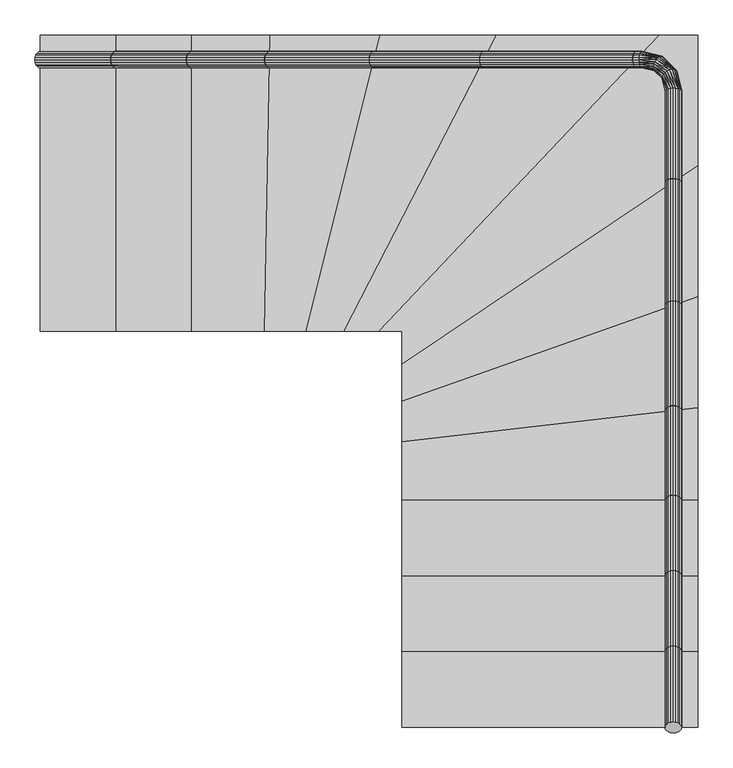
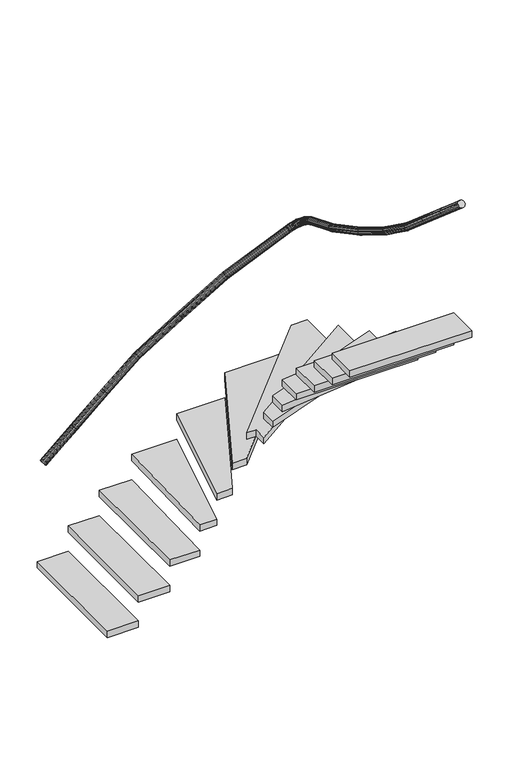
"""IFC4 building model written with IfcOpenShell, lengths in millimetres: stair geometry, 0_3d_modell."""

from ifc_helpers import new_model, si_unit, frame, origin, origin_with_axes, place, context, project, spatial, polyline, outline, extrude, faceted_brep, source, transform, mapped, element, save


def stair_1cae02e6(model_context):
    return source(origin(), model_context, "Body", "SolidModel", [
        extrude(outline(polyline([(1116.9018591, 1121.5036957), (2016.9018591, 1724.0707938), (2016.9018591, 1326.2140709), (1116.9018591, 1007.5896473), (1116.9018591, 1121.5036957)])), frame((0.0, 0.0, 1390.0), z_axis=(0.0, 0.0, 1.0), x_axis=(1.0, 0.0, 0.0)), (0.0, 0.0, 1.0), 50.0),
        extrude(outline(polyline([(1116.9018591, 476.9018591), (2016.9018591, 476.9018591), (2016.9018591, 246.9018591), (1116.9018591, 246.9018591), (1116.9018591, 476.9018591)])), frame((0.0, 0.0, 2184.2857143), z_axis=(0.0, 0.0, 1.0), x_axis=(1.0, 0.0, 0.0)), (0.0, 0.0, 1.0), 50.0),
        extrude(outline(polyline([(1.2235871, -7.9923214), (0.0, 0.0), (1.2235871, 7.9923214), (4.7745751, 15.2022986), (10.3053687, 20.9241691), (17.2745751, 24.5978359), (25.0, 25.8636953), (32.7254248, 24.5978359), (39.6946313, 20.9241691), (45.2254248, 15.2022986), (48.7764129, 7.9923214), (50.0, 0.0), (48.7764129, -7.9923214), (45.2254248, -15.2022986), (39.6946313, -20.924169), (32.7254248, -24.5978359), (25.0, -25.8636953), (17.2745751, -24.5978359), (10.3053687, -20.924169), (4.7745751, -15.2022986), (1.2235871, -7.9923214)])), frame((16.9018591, 2071.5036957, 869.5592366), z_axis=(0.7569287102857587, 0.0, 0.6534974579484897), x_axis=(0.0, -1.0, 0.0)), (0.0, 0.0, 1.0), 303.8595272),
        extrude(outline(polyline([(939.4821841, 1221.5036957), (1403.2627923, 2121.5036957), (1898.8029965, 2121.5036957), (1046.9018591, 1221.5036957), (939.4821841, 1221.5036957)])), frame((0.0, 0.0, 992.8571429), z_axis=(0.0, 0.0, 1.0), x_axis=(1.0, 0.0, 0.0)), (0.0, 0.0, 1.0), 50.0),
        faceted_brep([(1965.678272, 1303.6496314, 2465.062536), (1966.9018591, 1299.6620356, 2458.1306652), (1965.678272, 1295.6744399, 2451.1987943), (1962.127284, 1292.0771778, 2444.9454632), (1956.5964904, 1289.2223744, 2439.9827916), (1949.627284, 1287.3894778, 2436.7965603), (1941.9018591, 1286.7579047, 2435.6986598), (1934.1764343, 1287.3894778, 2436.7965603), (1927.2072278, 1289.2223744, 2439.9827916), (1921.6764343, 1292.0771778, 2444.9454632), (1918.1254462, 1295.6744399, 2451.1987943), (1916.9018591, 1299.6620356, 2458.1306652), (1918.1254462, 1303.6496314, 2465.062536), (1921.6764343, 1307.2468935, 2471.3158671), (1927.2072278, 1310.1016969, 2476.2785387), (1934.1764343, 1311.9345935, 2479.46477), (1941.9018591, 1312.5661666, 2480.5626705), (1949.627284, 1311.9345935, 2479.46477), (1956.5964904, 1310.1016969, 2476.2785387), (1962.127284, 1307.2468935, 2471.3158671), (1965.678272, 975.7637439, 2650.066583), (1966.9018591, 980.2280824, 2656.7020937), (1965.678272, 984.692421, 2663.3376045), (1962.127284, 988.719759, 2669.3235852), (1956.5964904, 991.9158725, 2674.0740863), (1949.627284, 993.9679037, 2677.1240958), (1941.9018591, 994.6749855, 2678.1750575), (1934.1764343, 993.9679037, 2677.1240958), (1927.2072278, 991.9158725, 2674.0740863), (1921.6764343, 988.719759, 2669.3235852), (1918.1254462, 984.692421, 2663.3376045), (1916.9018591, 980.2280824, 2656.7020937), (1918.1254462, 975.7637439, 2650.066583), (1921.6764343, 971.7364059, 2644.0806023), (1927.2072278, 968.5402924, 2639.3301012), (1934.1764343, 966.4882612, 2636.2800917), (1941.9018591, 965.7811794, 2635.22913), (1949.627284, 966.4882612, 2636.2800917), (1956.5964904, 968.5402924, 2639.3301012), (1962.127284, 971.7364059, 2644.0806023)], [[[0, 1, 2, 3, 4, 5, 6, 7, 8, 9, 10, 11, 12, 13, 14, 15, 16, 17, 18, 19]], [[20, 21, 22, 23, 24, 25, 26, 27, 28, 29, 30, 31, 32, 33, 34, 35, 36, 37, 38, 39]], [[21, 1, 0, 22]], [[22, 0, 19, 23]], [[23, 19, 18, 24]], [[24, 18, 17, 25]], [[25, 17, 16, 26]], [[26, 16, 15, 27]], [[27, 15, 14, 28]], [[28, 14, 13, 29]], [[29, 13, 12, 30]], [[30, 12, 11, 31]], [[31, 11, 10, 32]], [[32, 10, 9, 33]], [[33, 9, 8, 34]], [[34, 8, 7, 35]], [[35, 7, 6, 36]], [[36, 6, 5, 37]], [[37, 5, 4, 38]], [[38, 4, 3, 39]], [[39, 3, 2, 20]], [[20, 2, 1, 21]]]),
        extrude(outline(polyline([(1116.9018591, 884.9103911), (2016.9018591, 988.8933271), (2016.9018591, 706.9018591), (1116.9018591, 706.9018591), (1116.9018591, 884.9103911)])), frame((0.0, 0.0, 1787.1428571), z_axis=(0.0, 0.0, 1.0), x_axis=(1.0, 0.0, 0.0)), (0.0, 0.0, 1.0), 50.0),
        extrude(outline(polyline([(246.9018591, 1221.5036957), (246.9018591, 2121.5036957), (476.9018591, 2121.5036957), (476.9018591, 1221.5036957), (246.9018591, 1221.5036957)])), frame((0.0, 0.0, 198.5714286), z_axis=(0.0, 0.0, 1.0), x_axis=(1.0, 0.0, 0.0)), (0.0, 0.0, 1.0), 50.0),
        faceted_brep([(241.6788974, 2070.2801086, 1074.1802827), (246.9018591, 2071.5036957, 1068.1306652), (252.1248208, 2070.2801086, 1062.0810477), (256.8365226, 2066.7291206, 1056.6236089), (260.5757504, 2061.198327, 1052.2925609), (262.9764824, 2054.2291206, 1049.511857), (263.8037182, 2046.5036957, 1048.5536917), (262.9764824, 2038.7782709, 1049.511857), (260.5757504, 2031.8090644, 1052.2925609), (256.8365226, 2026.2782709, 1056.6236089), (252.1248208, 2022.7272828, 1062.0810477), (246.9018591, 2021.5036957, 1068.1306652), (241.6788974, 2022.7272828, 1074.1802827), (236.9671956, 2026.2782709, 1079.6377215), (233.2279679, 2031.8090644, 1083.9687694), (230.8272359, 2038.7782709, 1086.7494734), (230.0, 2046.5036957, 1087.7076387), (230.8272359, 2054.2291206, 1086.7494734), (233.2279679, 2061.198327, 1083.9687694), (236.9671956, 2066.7291206, 1079.6377215), (482.0819027, 2070.2801086, 1260.6154227), (476.9018591, 2071.5036957, 1266.7020937), (471.7218155, 2070.2801086, 1272.7887648), (467.0488307, 2066.7291206, 1278.2796301), (463.340329, 2061.198327, 1282.6372054), (460.9593243, 2054.2291206, 1285.434941), (460.138886, 2046.5036957, 1286.398975), (460.9593243, 2038.7782709, 1285.434941), (463.340329, 2031.8090644, 1282.6372054), (467.0488307, 2026.2782709, 1278.2796301), (471.7218155, 2022.7272828, 1272.7887648), (476.9018591, 2021.5036957, 1266.7020937), (482.0819027, 2022.7272828, 1260.6154227), (486.7548875, 2026.2782709, 1255.1245574), (490.4633893, 2031.8090644, 1250.7669821), (492.844394, 2038.7782709, 1247.9692465), (493.6648323, 2046.5036957, 1247.0052125), (492.844394, 2054.2291206, 1247.9692465), (490.4633893, 2061.198327, 1250.7669821), (486.7548875, 2066.7291206, 1255.1245574)], [[[0, 1, 2, 3, 4, 5, 6, 7, 8, 9, 10, 11, 12, 13, 14, 15, 16, 17, 18, 19]], [[20, 21, 22, 23, 24, 25, 26, 27, 28, 29, 30, 31, 32, 33, 34, 35, 36, 37, 38, 39]], [[21, 1, 0, 22]], [[22, 0, 19, 23]], [[23, 19, 18, 24]], [[24, 18, 17, 25]], [[25, 17, 16, 26]], [[26, 16, 15, 27]], [[27, 15, 14, 28]], [[28, 14, 13, 29]], [[29, 13, 12, 30]], [[30, 12, 11, 31]], [[31, 11, 10, 32]], [[32, 10, 9, 33]], [[33, 9, 8, 34]], [[34, 8, 7, 35]], [[35, 7, 6, 36]], [[36, 6, 5, 37]], [[37, 5, 4, 38]], [[38, 4, 3, 39]], [[39, 3, 2, 20]], [[20, 2, 1, 21]]]),
        extrude(outline(polyline([(1046.9018591, 1221.5036957), (1898.8029965, 2121.5036957), (2016.9018591, 2121.5036957), (2016.9018591, 1724.0707938), (1116.9018591, 1121.5036957), (1116.9018591, 1221.5036957), (1046.9018591, 1221.5036957)])), frame((0.0, 0.0, 1191.4285714), z_axis=(0.0, 0.0, 1.0), x_axis=(1.0, 0.0, 0.0)), (0.0, 0.0, 1.0), 50.0),
        extrude(outline(polyline([(1116.9018591, 706.9018591), (2016.9018591, 706.9018591), (2016.9018591, 476.9018591), (1116.9018591, 476.9018591), (1116.9018591, 706.9018591)])), frame((0.0, 0.0, 1985.7142857), z_axis=(0.0, 0.0, 1.0), x_axis=(1.0, 0.0, 0.0)), (0.0, 0.0, 1.0), 50.0),
        extrude(outline(polyline([(698.852304, 1221.5036957), (714.9514143, 2121.5036957), (1049.2205336, 2121.5036957), (824.5831846, 1221.5036957), (698.852304, 1221.5036957)])), frame((0.0, 0.0, 595.7142857), z_axis=(0.0, 0.0, 1.0), x_axis=(1.0, 0.0, 0.0)), (0.0, 0.0, 1.0), 50.0),
        extrude(outline(polyline([(16.9018591, 1221.5036957), (16.9018591, 2121.5036957), (246.9018591, 2121.5036957), (246.9018591, 1221.5036957), (16.9018591, 1221.5036957)])), origin_with_axes(), (0.0, 0.0, 1.0), 50.0),
        faceted_brep([(1360.9825862, 2070.2801086, 1869.5552099), (1364.6144083, 2071.5036957, 1862.4163795), (1368.2462303, 2070.2801086, 1855.277549), (1371.5225443, 2066.7291206, 1848.8375171), (1374.1226418, 2061.198327, 1843.7266788), (1375.7920071, 2054.2291206, 1840.4453186), (1376.3672312, 2046.5036957, 1839.3146389), (1375.7920071, 2038.7782709, 1840.4453186), (1374.1226418, 2031.8090644, 1843.7266788), (1371.5225443, 2026.2782709, 1848.8375171), (1368.2462303, 2022.7272828, 1855.277549), (1364.6144083, 2021.5036957, 1862.4163795), (1360.9825862, 2022.7272828, 1869.5552099), (1357.7062723, 2026.2782709, 1875.9952419), (1355.1061748, 2031.8090644, 1881.1060802), (1353.4368094, 2038.7782709, 1884.3874404), (1352.8615853, 2046.5036957, 1885.51812), (1353.4368094, 2054.2291206, 1884.3874404), (1355.1061748, 2061.198327, 1881.1060802), (1357.7062723, 2066.7291206, 1875.9952419), (1830.8955374, 2070.2801086, 2053.6142572), (1827.811235, 2071.5036957, 2060.987808), (1824.7269327, 2070.2801086, 2068.3613589), (1821.9445433, 2066.7291206, 2075.0131352), (1819.7364266, 2061.198327, 2080.2920148), (1818.3187285, 2054.2291206, 2083.6812642), (1817.830223, 2046.5036957, 2084.8491199), (1818.3187285, 2038.7782709, 2083.6812642), (1819.7364266, 2031.8090644, 2080.2920148), (1821.9445433, 2026.2782709, 2075.0131352), (1824.7269327, 2022.7272828, 2068.3613589), (1827.811235, 2021.5036957, 2060.987808), (1830.8955374, 2022.7272828, 2053.6142572), (1833.6779267, 2026.2782709, 2046.9624808), (1835.8860434, 2031.8090644, 2041.6836012), (1837.3037416, 2038.7782709, 2038.2943519), (1837.7922471, 2046.5036957, 2037.1264962), (1837.3037416, 2054.2291206, 2038.2943519), (1835.8860434, 2061.198327, 2041.6836012), (1833.6779267, 2066.7291206, 2046.9624808)], [[[0, 1, 2, 3, 4, 5, 6, 7, 8, 9, 10, 11, 12, 13, 14, 15, 16, 17, 18, 19]], [[20, 21, 22, 23, 24, 25, 26, 27, 28, 29, 30, 31, 32, 33, 34, 35, 36, 37, 38, 39]], [[21, 1, 0, 22]], [[22, 0, 19, 23]], [[23, 19, 18, 24]], [[24, 18, 17, 25]], [[25, 17, 16, 26]], [[26, 16, 15, 27]], [[27, 15, 14, 28]], [[28, 14, 13, 29]], [[29, 13, 12, 30]], [[30, 12, 11, 31]], [[31, 11, 10, 32]], [[32, 10, 9, 33]], [[33, 9, 8, 34]], [[34, 8, 7, 35]], [[35, 7, 6, 36]], [[36, 6, 5, 37]], [[37, 5, 4, 38]], [[38, 4, 3, 39]], [[39, 3, 2, 20]], [[20, 2, 1, 21]]]),
        extrude(outline(polyline([(476.9018591, 1221.5036957), (476.9018591, 2121.5036957), (714.9514143, 2121.5036957), (698.852304, 1221.5036957), (476.9018591, 1221.5036957)])), frame((0.0, 0.0, 397.1428571), z_axis=(0.0, 0.0, 1.0), x_axis=(1.0, 0.0, 0.0)), (0.0, 0.0, 1.0), 50.0),
        faceted_brep([(471.7218155, 2070.2801086, 1272.7887648), (476.9018591, 2071.5036957, 1266.7020937), (482.0819027, 2070.2801086, 1260.6154227), (486.7548875, 2066.7291206, 1255.1245574), (490.4633893, 2061.198327, 1250.7669821), (492.844394, 2054.2291206, 1247.9692465), (493.6648323, 2046.5036957, 1247.0052125), (492.844394, 2038.7782709, 1247.9692465), (490.4633893, 2031.8090644, 1250.7669821), (486.7548875, 2026.2782709, 1255.1245574), (482.0819027, 2022.7272828, 1260.6154227), (476.9018591, 2021.5036957, 1266.7020937), (471.7218155, 2022.7272828, 1272.7887648), (467.0488307, 2026.2782709, 1278.2796301), (463.340329, 2031.8090644, 1282.6372054), (460.9593243, 2038.7782709, 1285.434941), (460.138886, 2046.5036957, 1286.398975), (460.9593243, 2054.2291206, 1285.434941), (463.340329, 2061.198327, 1282.6372054), (467.0488307, 2066.7291206, 1278.2796301), (718.3225173, 2070.2801086, 1458.7947987), (713.6098217, 2071.5036957, 1465.2735223), (708.8971261, 2070.2801086, 1471.7522459), (704.645742, 2066.7291206, 1477.5967869), (701.2718245, 2061.198327, 1482.2350408), (699.1056361, 2054.2291206, 1485.2129832), (698.3592184, 2046.5036957, 1486.2391122), (699.1056361, 2038.7782709, 1485.2129832), (701.2718245, 2031.8090644, 1482.2350408), (704.645742, 2026.2782709, 1477.5967869), (708.8971261, 2022.7272828, 1471.7522459), (713.6098217, 2021.5036957, 1465.2735223), (718.3225173, 2022.7272828, 1458.7947987), (722.5739015, 2026.2782709, 1452.9502578), (725.947819, 2031.8090644, 1448.3120038), (728.1140074, 2038.7782709, 1445.3340614), (728.8604251, 2046.5036957, 1444.3079324), (728.1140074, 2054.2291206, 1445.3340614), (725.947819, 2061.198327, 1448.3120038), (722.5739015, 2066.7291206, 1452.9502578)], [[[0, 1, 2, 3, 4, 5, 6, 7, 8, 9, 10, 11, 12, 13, 14, 15, 16, 17, 18, 19]], [[20, 21, 22, 23, 24, 25, 26, 27, 28, 29, 30, 31, 32, 33, 34, 35, 36, 37, 38, 39]], [[21, 1, 0, 22]], [[22, 0, 19, 23]], [[23, 19, 18, 24]], [[24, 18, 17, 25]], [[25, 17, 16, 26]], [[26, 16, 15, 27]], [[27, 15, 14, 28]], [[28, 14, 13, 29]], [[29, 13, 12, 30]], [[30, 12, 11, 31]], [[31, 11, 10, 32]], [[32, 10, 9, 33]], [[33, 9, 8, 34]], [[34, 8, 7, 35]], [[35, 7, 6, 36]], [[36, 6, 5, 37]], [[37, 5, 4, 38]], [[38, 4, 3, 39]], [[39, 3, 2, 20]], [[20, 2, 1, 21]]]),
        faceted_brep([(1965.678272, 984.692421, 2663.3376045), (1966.9018591, 980.2280824, 2656.7020937), (1965.678272, 975.7637439, 2650.066583), (1962.127284, 971.7364059, 2644.0806023), (1956.5964904, 968.5402924, 2639.3301012), (1949.627284, 966.4882612, 2636.2800917), (1941.9018591, 965.7811794, 2635.22913), (1934.1764343, 966.4882612, 2636.2800917), (1927.2072278, 968.5402924, 2639.3301012), (1921.6764343, 971.7364059, 2644.0806023), (1918.1254462, 975.7637439, 2650.066583), (1916.9018591, 980.2280824, 2656.7020937), (1918.1254462, 984.692421, 2663.3376045), (1921.6764343, 988.719759, 2669.3235852), (1927.2072278, 991.9158725, 2674.0740863), (1934.1764343, 993.9679037, 2677.1240958), (1941.9018591, 994.6749855, 2678.1750575), (1949.627284, 993.9679037, 2677.1240958), (1956.5964904, 991.9158725, 2674.0740863), (1962.127284, 988.719759, 2669.3235852), (1965.678272, 701.932844, 2849.004659), (1966.9018591, 706.9018591, 2855.2735223), (1965.678272, 711.8708742, 2861.5423857), (1962.127284, 716.3534875, 2867.197609), (1956.5964904, 719.9109095, 2871.6856196), (1949.627284, 722.194915, 2874.5670998), (1941.9018591, 722.9819297, 2875.5599903), (1934.1764343, 722.194915, 2874.5670998), (1927.2072278, 719.9109095, 2871.6856196), (1921.6764343, 716.3534875, 2867.197609), (1918.1254462, 711.8708742, 2861.5423857), (1916.9018591, 706.9018591, 2855.2735223), (1918.1254462, 701.932844, 2849.004659), (1921.6764343, 697.4502308, 2843.3494356), (1927.2072278, 693.8928087, 2838.861425), (1934.1764343, 691.6088032, 2835.9799448), (1941.9018591, 690.8217885, 2834.9870544), (1949.627284, 691.6088032, 2835.9799448), (1956.5964904, 693.8928087, 2838.861425), (1962.127284, 697.4502308, 2843.3494356)], [[[0, 1, 2, 3, 4, 5, 6, 7, 8, 9, 10, 11, 12, 13, 14, 15, 16, 17, 18, 19]], [[20, 21, 22, 23, 24, 25, 26, 27, 28, 29, 30, 31, 32, 33, 34, 35, 36, 37, 38, 39]], [[21, 1, 0, 22]], [[22, 0, 19, 23]], [[23, 19, 18, 24]], [[24, 18, 17, 25]], [[25, 17, 16, 26]], [[26, 16, 15, 27]], [[27, 15, 14, 28]], [[28, 14, 13, 29]], [[29, 13, 12, 30]], [[30, 12, 11, 31]], [[31, 11, 10, 32]], [[32, 10, 9, 33]], [[33, 9, 8, 34]], [[34, 8, 7, 35]], [[35, 7, 6, 36]], [[36, 6, 5, 37]], [[37, 5, 4, 38]], [[38, 4, 3, 39]], [[39, 3, 2, 20]], [[20, 2, 1, 21]]]),
        extrude(outline(polyline([(1.2235871, -7.9923214), (0.0, 0.0), (1.2235871, 7.9923214), (4.7745751, 15.2022986), (10.3053687, 20.924169), (17.2745751, 24.597836), (25.0, 25.8636953), (32.7254248, 24.597836), (39.6946313, 20.924169), (45.2254248, 15.2022986), (48.7764129, 7.9923214), (50.0, 0.0), (48.7764129, -7.9923214), (45.2254248, -15.2022986), (39.6946313, -20.924169), (32.7254248, -24.5978359), (25.0, -25.8636953), (17.2745751, -24.5978359), (10.3053687, -20.924169), (4.7745751, -15.2022986), (1.2235871, -7.9923214)])), frame((1966.9018591, 246.9018591, 3252.4163795), z_axis=(0.0, -0.7569287102857001, 0.6534974579485575), x_axis=(-1.0, 0.0, 0.0)), (0.0, 0.0, 1.0), 303.8595272),
        faceted_brep([(1026.3366143, 2070.2801086, 1670.6674124), (1030.5007545, 2071.5036957, 1663.8449509), (1034.6648948, 2070.2801086, 1657.0224894), (1038.42142, 2066.7291206, 1650.867858), (1041.4026152, 2061.198327, 1645.9835149), (1043.3166604, 2054.2291206, 1642.8475735), (1043.9761954, 2046.5036957, 1641.7670018), (1043.3166604, 2038.7782709, 1642.8475735), (1041.4026152, 2031.8090644, 1645.9835149), (1038.42142, 2026.2782709, 1650.867858), (1034.6648948, 2022.7272828, 1657.0224894), (1030.5007545, 2021.5036957, 1663.8449509), (1026.3366143, 2022.7272828, 1670.6674124), (1022.5800891, 2026.2782709, 1676.8220438), (1019.5988939, 2031.8090644, 1681.7063869), (1017.6848487, 2038.7782709, 1684.8423282), (1017.0253137, 2046.5036957, 1685.9229), (1017.6848487, 2054.2291206, 1684.8423282), (1019.5988939, 2061.198327, 1681.7063869), (1022.5800891, 2066.7291206, 1676.8220438), (1368.2462303, 2070.2801086, 1855.277549), (1364.6144083, 2071.5036957, 1862.4163795), (1360.9825862, 2070.2801086, 1869.5552099), (1357.7062723, 2066.7291206, 1875.9952419), (1355.1061748, 2061.198327, 1881.1060802), (1353.4368094, 2054.2291206, 1884.3874404), (1352.8615853, 2046.5036957, 1885.51812), (1353.4368094, 2038.7782709, 1884.3874404), (1355.1061748, 2031.8090644, 1881.1060802), (1357.7062723, 2026.2782709, 1875.9952419), (1360.9825862, 2022.7272828, 1869.5552099), (1364.6144083, 2021.5036957, 1862.4163795), (1368.2462303, 2022.7272828, 1855.277549), (1371.5225443, 2026.2782709, 1848.8375171), (1374.1226418, 2031.8090644, 1843.7266788), (1375.7920071, 2038.7782709, 1840.4453186), (1376.3672312, 2046.5036957, 1839.3146389), (1375.7920071, 2054.2291206, 1840.4453186), (1374.1226418, 2061.198327, 1843.7266788), (1371.5225443, 2066.7291206, 1848.8375171)], [[[0, 1, 2, 3, 4, 5, 6, 7, 8, 9, 10, 11, 12, 13, 14, 15, 16, 17, 18, 19]], [[20, 21, 22, 23, 24, 25, 26, 27, 28, 29, 30, 31, 32, 33, 34, 35, 36, 37, 38, 39]], [[21, 1, 0, 22]], [[22, 0, 19, 23]], [[23, 19, 18, 24]], [[24, 18, 17, 25]], [[25, 17, 16, 26]], [[26, 16, 15, 27]], [[27, 15, 14, 28]], [[28, 14, 13, 29]], [[29, 13, 12, 30]], [[30, 12, 11, 31]], [[31, 11, 10, 32]], [[32, 10, 9, 33]], [[33, 9, 8, 34]], [[34, 8, 7, 35]], [[35, 7, 6, 36]], [[36, 6, 5, 37]], [[37, 5, 4, 38]], [[38, 4, 3, 39]], [[39, 3, 2, 20]], [[20, 2, 1, 21]]]),
        extrude(outline(polyline([(1116.9018591, 1007.5896473), (2016.9018591, 1326.2140709), (2016.9018591, 988.8933271), (1116.9018591, 884.9103911), (1116.9018591, 1007.5896473)])), frame((0.0, 0.0, 1588.5714286), z_axis=(0.0, 0.0, 1.0), x_axis=(1.0, 0.0, 0.0)), (0.0, 0.0, 1.0), 50.0),
        faceted_brep([(1824.7269327, 2070.2801086, 2068.3613589), (1827.811235, 2071.5036957, 2060.987808), (1830.8955374, 2070.2801086, 2053.6142572), (1833.6779267, 2066.7291206, 2046.9624808), (1835.8860434, 2061.198327, 2041.6836012), (1837.3037416, 2054.2291206, 2038.2943519), (1837.7922471, 2046.5036957, 2037.1264962), (1837.3037416, 2038.7782709, 2038.2943519), (1835.8860434, 2031.8090644, 2041.6836012), (1833.6779267, 2026.2782709, 2046.9624808), (1830.8955374, 2022.7272828, 2053.6142572), (1827.811235, 2021.5036957, 2060.987808), (1824.7269327, 2022.7272828, 2068.3613589), (1821.9445433, 2026.2782709, 2075.0131352), (1819.7364266, 2031.8090644, 2080.2920148), (1818.3187285, 2038.7782709, 2083.6812642), (1817.830223, 2046.5036957, 2084.8491199), (1818.3187285, 2054.2291206, 2083.6812642), (1819.7364266, 2061.198327, 2080.2920148), (1821.9445433, 2066.7291206, 2075.0131352), (1965.678272, 1670.4655995, 2252.3109173), (1966.9018591, 1673.856869, 2259.5592366), (1965.678272, 1677.2481385, 2266.8075559), (1962.127284, 1680.3074469, 2273.3463592), (1956.5964904, 1682.7353278, 2278.5355829), (1949.627284, 1684.2941233, 2281.8672695), (1941.9018591, 1684.8312476, 2283.0152905), (1934.1764343, 1684.2941233, 2281.8672695), (1927.2072278, 1682.7353278, 2278.5355829), (1921.6764343, 1680.3074469, 2273.3463592), (1918.1254462, 1677.2481385, 2266.8075559), (1916.9018591, 1673.856869, 2259.5592366), (1918.1254462, 1670.4655995, 2252.3109173), (1921.6764343, 1667.4062911, 2245.772114), (1927.2072278, 1664.9784102, 2240.5828904), (1934.1764343, 1663.4196147, 2237.2512037), (1941.9018591, 1662.8824904, 2236.1031827), (1949.627284, 1663.4196147, 2237.2512037), (1956.5964904, 1664.9784102, 2240.5828904), (1962.127284, 1667.4062911, 2245.772114), (1846.1118218, 2071.5036957, 2068.4537913), (1843.0928107, 2070.2801086, 2075.8539787), (1840.3693214, 2066.7291206, 2082.5297841), (1838.2079481, 2061.198327, 2087.8277333), (1836.820261, 2054.2291206, 2091.2292261), (1836.3420966, 2046.5036957, 2092.4013006), (1836.820261, 2038.7782709, 2091.2292261), (1838.2079481, 2031.8090644, 2087.8277333), (1840.3693214, 2026.2782709, 2082.5297841), (1843.0928107, 2022.7272828, 2075.8539787), (1846.1118218, 2021.5036957, 2068.4537913), (1849.1308329, 2022.7272828, 2061.053604), (1851.8543222, 2026.2782709, 2054.3777985), (1854.0156955, 2031.8090644, 2049.0798493), (1855.4033826, 2038.7782709, 2045.6783565), (1855.881547, 2046.5036957, 2044.506282), (1855.4033826, 2054.2291206, 2045.6783565), (1854.0156955, 2061.198327, 2049.0798493), (1851.8543222, 2066.7291206, 2054.3777985), (1849.1308329, 2070.2801086, 2061.053604), (1908.6788758, 2056.4792109, 2093.9682441), (1904.6951215, 2057.2618667, 2100.9604911), (1899.9277994, 2055.8204705, 2107.2682883), (1894.8435681, 2052.2961161, 2112.2741844), (1889.9401076, 2047.0337921, 2115.4881676), (1885.6974028, 2040.5486112, 2116.5956307), (1882.5307592, 2033.4753883, 2115.4881676), (1880.7501499, 2026.5064996, 2112.2741844), (1880.5298735, 2020.3241085, 2107.2682883), (1881.8914919, 2015.5333905, 2100.9604911), (1884.7017207, 2012.6032946, 2093.9682441), (1888.685475, 2011.8206388, 2086.9759971), (1893.4527971, 2013.262035, 2080.6681999), (1898.5370284, 2016.7863894, 2075.6623037), (1903.4404889, 2022.0487134, 2072.4483206), (1907.6831937, 2028.5338943, 2071.3408574), (1910.8498373, 2035.6071172, 2072.4483206), (1912.6304465, 2042.5760059, 2075.6623037), (1912.850723, 2048.758397, 2080.6681999), (1911.4891045, 2053.549115, 2086.9759971), (1951.8773743, 2013.2807124, 2121.0971401), (1948.9472784, 2016.0909411, 2128.0893871), (1944.1565604, 2017.4525596, 2134.3971843), (1937.9741693, 2017.2322831, 2139.4030804), (1931.0052806, 2015.4516739, 2142.6170636), (1923.9320577, 2012.2850303, 2143.7245267), (1917.4468768, 2008.0423255, 2142.6170636), (1912.1845528, 2003.138865, 2139.4030804), (1908.6601984, 1998.0546337, 2134.3971843), (1907.2188022, 1993.2873116, 2128.0893871), (1908.001458, 1989.3035573, 2121.0971401), (1910.9315539, 1986.4933285, 2114.1048931), (1915.7222719, 1985.1317101, 2107.7970959), (1921.904663, 1985.3519865, 2102.7911997), (1928.8735517, 1987.1325958, 2099.5772166), (1935.9467746, 1990.2992394, 2098.4697534), (1942.4319555, 1994.5419442, 2099.5772166), (1947.6942795, 1999.4454047, 2102.7911997), (1951.2186339, 2004.529636, 2107.7970959), (1952.6600301, 2009.2969581, 2114.1048931), (1966.9018591, 1950.7136584, 2146.6115929), (1965.678272, 1953.7326696, 2154.0117802), (1962.127284, 1956.4561588, 2160.6875857), (1956.5964904, 1958.6175321, 2165.9855349), (1949.627284, 1960.0052192, 2169.3870277), (1941.9018591, 1960.4833836, 2170.5591022), (1934.1764343, 1960.0052192, 2169.3870277), (1927.2072278, 1958.6175321, 2165.9855349), (1921.6764343, 1956.4561588, 2160.6875857), (1918.1254462, 1953.7326696, 2154.0117802), (1916.9018591, 1950.7136584, 2146.6115929), (1918.1254462, 1947.6946473, 2139.2114055), (1921.6764343, 1944.971158, 2132.5356001), (1927.2072278, 1942.8097847, 2127.2376509), (1934.1764343, 1941.4220976, 2123.8361581), (1941.9018591, 1940.9439332, 2122.6640835), (1949.627284, 1941.4220976, 2123.8361581), (1956.5964904, 1942.8097847, 2127.2376509), (1962.127284, 1944.971158, 2132.5356001), (1965.678272, 1947.6946473, 2139.2114055)], [[[0, 1, 2, 3, 4, 5, 6, 7, 8, 9, 10, 11, 12, 13, 14, 15, 16, 17, 18, 19]], [[20, 21, 22, 23, 24, 25, 26, 27, 28, 29, 30, 31, 32, 33, 34, 35, 36, 37, 38, 39]], [[40, 1, 0, 41]], [[41, 0, 19, 42]], [[42, 19, 18, 43]], [[43, 18, 17, 44]], [[44, 17, 16, 45]], [[45, 16, 15, 46]], [[46, 15, 14, 47]], [[47, 14, 13, 48]], [[48, 13, 12, 49]], [[49, 12, 11, 50]], [[50, 11, 10, 51]], [[51, 10, 9, 52]], [[52, 9, 8, 53]], [[53, 8, 7, 54]], [[54, 7, 6, 55]], [[55, 6, 5, 56]], [[56, 5, 4, 57]], [[57, 4, 3, 58]], [[58, 3, 2, 59]], [[59, 2, 1, 40]], [[60, 40, 41]], [[60, 41, 61]], [[61, 41, 42]], [[61, 42, 62]], [[62, 42, 43]], [[62, 43, 63]], [[63, 43, 44]], [[63, 44, 64]], [[64, 44, 45]], [[64, 45, 65]], [[65, 45, 46]], [[65, 46, 66]], [[66, 46, 47]], [[66, 47, 67]], [[67, 47, 48]], [[67, 48, 68]], [[68, 48, 49]], [[68, 49, 69]], [[69, 49, 50]], [[69, 50, 70]], [[70, 50, 51]], [[70, 51, 71]], [[71, 51, 52]], [[71, 52, 72]], [[72, 52, 53]], [[72, 53, 73]], [[73, 53, 54]], [[73, 54, 74]], [[74, 54, 55]], [[74, 55, 75]], [[75, 55, 56]], [[75, 56, 76]], [[76, 56, 57]], [[76, 57, 77]], [[77, 57, 58]], [[77, 58, 78]], [[78, 58, 59]], [[78, 59, 79]], [[79, 59, 40]], [[79, 40, 60]], [[80, 60, 61]], [[80, 61, 81]], [[81, 61, 62]], [[81, 62, 82]], [[82, 62, 63]], [[82, 63, 83]], [[83, 63, 64]], [[83, 64, 84]], [[84, 64, 65]], [[84, 65, 85]], [[85, 65, 66]], [[85, 66, 86]], [[86, 66, 67]], [[86, 67, 87]], [[87, 67, 68]], [[87, 68, 88]], [[88, 68, 69]], [[88, 69, 89]], [[89, 69, 70]], [[89, 70, 90]], [[90, 70, 71]], [[90, 71, 91]], [[91, 71, 72]], [[91, 72, 92]], [[92, 72, 73]], [[92, 73, 93]], [[93, 73, 74]], [[93, 74, 94]], [[94, 74, 75]], [[94, 75, 95]], [[95, 75, 76]], [[95, 76, 96]], [[96, 76, 77]], [[96, 77, 97]], [[97, 77, 78]], [[97, 78, 98]], [[98, 78, 79]], [[98, 79, 99]], [[99, 79, 60]], [[99, 60, 80]], [[100, 80, 81]], [[100, 81, 101]], [[101, 81, 82]], [[101, 82, 102]], [[102, 82, 83]], [[102, 83, 103]], [[103, 83, 84]], [[103, 84, 104]], [[104, 84, 85]], [[104, 85, 105]], [[105, 85, 86]], [[105, 86, 106]], [[106, 86, 87]], [[106, 87, 107]], [[107, 87, 88]], [[107, 88, 108]], [[108, 88, 89]], [[108, 89, 109]], [[109, 89, 90]], [[109, 90, 110]], [[110, 90, 91]], [[110, 91, 111]], [[111, 91, 92]], [[111, 92, 112]], [[112, 92, 93]], [[112, 93, 113]], [[113, 93, 94]], [[113, 94, 114]], [[114, 94, 95]], [[114, 95, 115]], [[115, 95, 96]], [[115, 96, 116]], [[116, 96, 97]], [[116, 97, 117]], [[117, 97, 98]], [[117, 98, 118]], [[118, 98, 99]], [[118, 99, 119]], [[119, 99, 80]], [[119, 80, 100]], [[21, 100, 101, 22]], [[22, 101, 102, 23]], [[23, 102, 103, 24]], [[24, 103, 104, 25]], [[25, 104, 105, 26]], [[26, 105, 106, 27]], [[27, 106, 107, 28]], [[28, 107, 108, 29]], [[29, 108, 109, 30]], [[30, 109, 110, 31]], [[31, 110, 111, 32]], [[32, 111, 112, 33]], [[33, 112, 113, 34]], [[34, 113, 114, 35]], [[35, 114, 115, 36]], [[36, 115, 116, 37]], [[37, 116, 117, 38]], [[38, 117, 118, 39]], [[39, 118, 119, 20]], [[20, 119, 100, 21]]]),
        faceted_brep([(1965.678272, 1677.2481385, 2266.8075559), (1966.9018591, 1673.856869, 2259.5592366), (1965.678272, 1670.4655995, 2252.3109173), (1962.127284, 1667.4062911, 2245.772114), (1956.5964904, 1664.9784102, 2240.5828904), (1949.627284, 1663.4196147, 2237.2512037), (1941.9018591, 1662.8824904, 2236.1031827), (1934.1764343, 1663.4196147, 2237.2512037), (1927.2072278, 1664.9784102, 2240.5828904), (1921.6764343, 1667.4062911, 2245.772114), (1918.1254462, 1670.4655995, 2252.3109173), (1916.9018591, 1673.856869, 2259.5592366), (1918.1254462, 1677.2481385, 2266.8075559), (1921.6764343, 1680.3074469, 2273.3463592), (1927.2072278, 1682.7353278, 2278.5355829), (1934.1764343, 1684.2941233, 2281.8672695), (1941.9018591, 1684.8312476, 2283.0152905), (1949.627284, 1684.2941233, 2281.8672695), (1956.5964904, 1682.7353278, 2278.5355829), (1962.127284, 1680.3074469, 2273.3463592), (1965.678272, 1295.6744399, 2451.1987943), (1966.9018591, 1299.6620356, 2458.1306652), (1965.678272, 1303.6496314, 2465.062536), (1962.127284, 1307.2468935, 2471.3158671), (1956.5964904, 1310.1016969, 2476.2785387), (1949.627284, 1311.9345935, 2479.46477), (1941.9018591, 1312.5661666, 2480.5626705), (1934.1764343, 1311.9345935, 2479.46477), (1927.2072278, 1310.1016969, 2476.2785387), (1921.6764343, 1307.2468935, 2471.3158671), (1918.1254462, 1303.6496314, 2465.062536), (1916.9018591, 1299.6620356, 2458.1306652), (1918.1254462, 1295.6744399, 2451.1987943), (1921.6764343, 1292.0771778, 2444.9454632), (1927.2072278, 1289.2223744, 2439.9827916), (1934.1764343, 1287.3894778, 2436.7965603), (1941.9018591, 1286.7579047, 2435.6986598), (1949.627284, 1287.3894778, 2436.7965603), (1956.5964904, 1289.2223744, 2439.9827916), (1962.127284, 1292.0771778, 2444.9454632)], [[[0, 1, 2, 3, 4, 5, 6, 7, 8, 9, 10, 11, 12, 13, 14, 15, 16, 17, 18, 19]], [[20, 21, 22, 23, 24, 25, 26, 27, 28, 29, 30, 31, 32, 33, 34, 35, 36, 37, 38, 39]], [[21, 1, 0, 22]], [[22, 0, 19, 23]], [[23, 19, 18, 24]], [[24, 18, 17, 25]], [[25, 17, 16, 26]], [[26, 16, 15, 27]], [[27, 15, 14, 28]], [[28, 14, 13, 29]], [[29, 13, 12, 30]], [[30, 12, 11, 31]], [[31, 11, 10, 32]], [[32, 10, 9, 33]], [[33, 9, 8, 34]], [[34, 8, 7, 35]], [[35, 7, 6, 36]], [[36, 6, 5, 37]], [[37, 5, 4, 38]], [[38, 4, 3, 39]], [[39, 3, 2, 20]], [[20, 2, 1, 21]]]),
        extrude(outline(polyline([(824.5831846, 1221.5036957), (1049.2205336, 2121.5036957), (1403.2627923, 2121.5036957), (939.4821841, 1221.5036957), (824.5831846, 1221.5036957)])), frame((0.0, 0.0, 794.2857143), z_axis=(0.0, 0.0, 1.0), x_axis=(1.0, 0.0, 0.0)), (0.0, 0.0, 1.0), 50.0),
        extrude(outline(polyline([(1.2235871, -7.9923214), (0.0, 0.0), (1.2235871, 7.9923214), (4.7745751, 15.2022986), (10.3053687, 20.924169), (17.2745751, 24.5978359), (25.0, 25.8636953), (32.7254248, 24.5978359), (39.6946313, 20.924169), (45.2254248, 15.2022986), (48.7764129, 7.9923214), (50.0, 0.0), (48.7764129, -7.9923214), (45.2254248, -15.2022986), (39.6946313, -20.9241691), (32.7254248, -24.5978359), (25.0, -25.8636953), (17.2745751, -24.5978359), (10.3053687, -20.9241691), (4.7745751, -15.2022986), (1.2235871, -7.9923214)])), frame((1966.9018591, 476.9018591, 3053.8449509), z_axis=(0.0, -0.7569287102856936, 0.6534974579485651), x_axis=(-1.0, 0.0, 0.0)), (0.0, 0.0, 1.0), 303.8595272),
        faceted_brep([(708.8971261, 2070.2801086, 1471.7522459), (713.6098217, 2071.5036957, 1465.2735223), (718.3225173, 2070.2801086, 1458.7947987), (722.5739015, 2066.7291206, 1452.9502578), (725.947819, 2061.198327, 1448.3120038), (728.1140074, 2054.2291206, 1445.3340614), (728.8604251, 2046.5036957, 1444.3079324), (728.1140074, 2038.7782709, 1445.3340614), (725.947819, 2031.8090644, 1448.3120038), (722.5739015, 2026.2782709, 1452.9502578), (718.3225173, 2022.7272828, 1458.7947987), (713.6098217, 2021.5036957, 1465.2735223), (708.8971261, 2022.7272828, 1471.7522459), (704.645742, 2026.2782709, 1477.5967869), (701.2718245, 2031.8090644, 1482.2350408), (699.1056361, 2038.7782709, 1485.2129832), (698.3592184, 2046.5036957, 1486.2391122), (699.1056361, 2054.2291206, 1485.2129832), (701.2718245, 2061.198327, 1482.2350408), (704.645742, 2066.7291206, 1477.5967869), (1034.6648948, 2070.2801086, 1657.0224894), (1030.5007545, 2071.5036957, 1663.8449509), (1026.3366143, 2070.2801086, 1670.6674124), (1022.5800891, 2066.7291206, 1676.8220438), (1019.5988939, 2061.198327, 1681.7063869), (1017.6848487, 2054.2291206, 1684.8423282), (1017.0253137, 2046.5036957, 1685.9229), (1017.6848487, 2038.7782709, 1684.8423282), (1019.5988939, 2031.8090644, 1681.7063869), (1022.5800891, 2026.2782709, 1676.8220438), (1026.3366143, 2022.7272828, 1670.6674124), (1030.5007545, 2021.5036957, 1663.8449509), (1034.6648948, 2022.7272828, 1657.0224894), (1038.42142, 2026.2782709, 1650.867858), (1041.4026152, 2031.8090644, 1645.9835149), (1043.3166604, 2038.7782709, 1642.8475735), (1043.9761954, 2046.5036957, 1641.7670018), (1043.3166604, 2054.2291206, 1642.8475735), (1041.4026152, 2061.198327, 1645.9835149), (1038.42142, 2066.7291206, 1650.867858)], [[[0, 1, 2, 3, 4, 5, 6, 7, 8, 9, 10, 11, 12, 13, 14, 15, 16, 17, 18, 19]], [[20, 21, 22, 23, 24, 25, 26, 27, 28, 29, 30, 31, 32, 33, 34, 35, 36, 37, 38, 39]], [[21, 1, 0, 22]], [[22, 0, 19, 23]], [[23, 19, 18, 24]], [[24, 18, 17, 25]], [[25, 17, 16, 26]], [[26, 16, 15, 27]], [[27, 15, 14, 28]], [[28, 14, 13, 29]], [[29, 13, 12, 30]], [[30, 12, 11, 31]], [[31, 11, 10, 32]], [[32, 10, 9, 33]], [[33, 9, 8, 34]], [[34, 8, 7, 35]], [[35, 7, 6, 36]], [[36, 6, 5, 37]], [[37, 5, 4, 38]], [[38, 4, 3, 39]], [[39, 3, 2, 20]], [[20, 2, 1, 21]]]),
        faceted_brep([(1965.678272, 711.8708742, 2861.5423857), (1966.9018591, 706.9018591, 2855.2735223), (1965.678272, 701.932844, 2849.004659), (1962.127284, 697.4502308, 2843.3494356), (1956.5964904, 693.8928087, 2838.861425), (1949.627284, 691.6088032, 2835.9799448), (1941.9018591, 690.8217885, 2834.9870544), (1934.1764343, 691.6088032, 2835.9799448), (1927.2072278, 693.8928087, 2838.861425), (1921.6764343, 697.4502308, 2843.3494356), (1918.1254462, 701.932844, 2849.004659), (1916.9018591, 706.9018591, 2855.2735223), (1918.1254462, 711.8708742, 2861.5423857), (1921.6764343, 716.3534875, 2867.197609), (1927.2072278, 719.9109095, 2871.6856196), (1934.1764343, 722.194915, 2874.5670998), (1941.9018591, 722.9819297, 2875.5599903), (1949.627284, 722.194915, 2874.5670998), (1956.5964904, 719.9109095, 2871.6856196), (1962.127284, 716.3534875, 2867.197609), (1965.678272, 471.6788974, 3047.7953334), (1966.9018591, 476.9018591, 3053.8449509), (1965.678272, 482.1248208, 3059.8945684), (1962.127284, 486.8365226, 3065.3520072), (1956.5964904, 490.5757504, 3069.6830552), (1949.627284, 492.9764824, 3072.4637591), (1941.9018591, 493.8037182, 3073.4219244), (1934.1764343, 492.9764824, 3072.4637591), (1927.2072278, 490.5757504, 3069.6830552), (1921.6764343, 486.8365226, 3065.3520072), (1918.1254462, 482.1248208, 3059.8945684), (1916.9018591, 476.9018591, 3053.8449509), (1918.1254462, 471.6788974, 3047.7953334), (1921.6764343, 466.9671956, 3042.3378946), (1927.2072278, 463.2279679, 3038.0068466), (1934.1764343, 460.8272359, 3035.2261427), (1941.9018591, 460.0, 3034.2679774), (1949.627284, 460.8272359, 3035.2261427), (1956.5964904, 463.2279679, 3038.0068466), (1962.127284, 466.9671956, 3042.3378946)], [[[0, 1, 2, 3, 4, 5, 6, 7, 8, 9, 10, 11, 12, 13, 14, 15, 16, 17, 18, 19]], [[20, 21, 22, 23, 24, 25, 26, 27, 28, 29, 30, 31, 32, 33, 34, 35, 36, 37, 38, 39]], [[21, 1, 0, 22]], [[22, 0, 19, 23]], [[23, 19, 18, 24]], [[24, 18, 17, 25]], [[25, 17, 16, 26]], [[26, 16, 15, 27]], [[27, 15, 14, 28]], [[28, 14, 13, 29]], [[29, 13, 12, 30]], [[30, 12, 11, 31]], [[31, 11, 10, 32]], [[32, 10, 9, 33]], [[33, 9, 8, 34]], [[34, 8, 7, 35]], [[35, 7, 6, 36]], [[36, 6, 5, 37]], [[37, 5, 4, 38]], [[38, 4, 3, 39]], [[39, 3, 2, 20]], [[20, 2, 1, 21]]]),
        extrude(outline(polyline([(1116.9018591, 246.9018591), (2016.9018591, 246.9018591), (2016.9018591, 16.9018591), (1116.9018591, 16.9018591), (1116.9018591, 246.9018591)])), frame((0.0, 0.0, 2382.8571429), z_axis=(0.0, 0.0, 1.0), x_axis=(1.0, 0.0, 0.0)), (0.0, 0.0, 1.0), 50.0),
    ])


if __name__ == "__main__":
    model = new_model("IFC4")
    model_context = context("Model", 3, world=origin())
    ifc_project = project(units=[si_unit("LENGTHUNIT", "METRE", prefix="MILLI")], contexts=[model_context])
    site = spatial("IfcSite", under=ifc_project)
    building = spatial("IfcBuilding", under=site)
    placement = place(None, origin())
    stair_shape = stair_1cae02e6(model_context)
    element("IfcStair", 1, ObjectType="0_3d_modell", at=placement, inside=building, context=model_context, shape_type="MappedRepresentation", body=[
        mapped(stair_shape, transform((0.0, 0.0, 0.0), x_axis=(1.0, 0.0, 0.0), y_axis=(0.0, 1.0, 0.0), z_axis=(0.0, 0.0, 1.0))),
    ])
    save(model, "model.ifc")

# Revit data of these elements
# Element 1 (IfcStair, "0_3d_modell")
#   Materials on its faces: "*1", "weiss"
# Materials
#   "*1": class "Unassigned", colour RGB 175 175 175, transparency 0
#   "weiss": class "Unassigned", colour RGB 255 255 255, transparency 0
